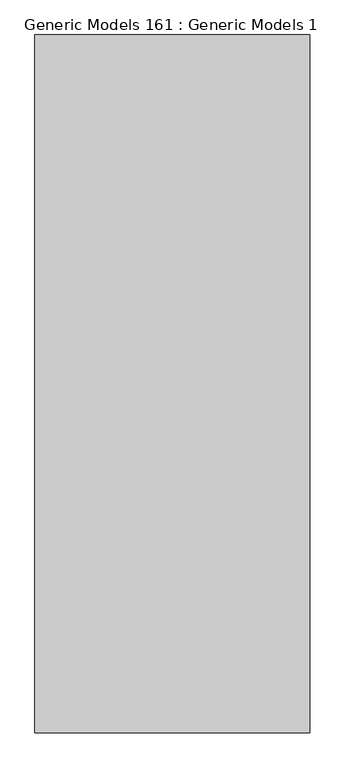
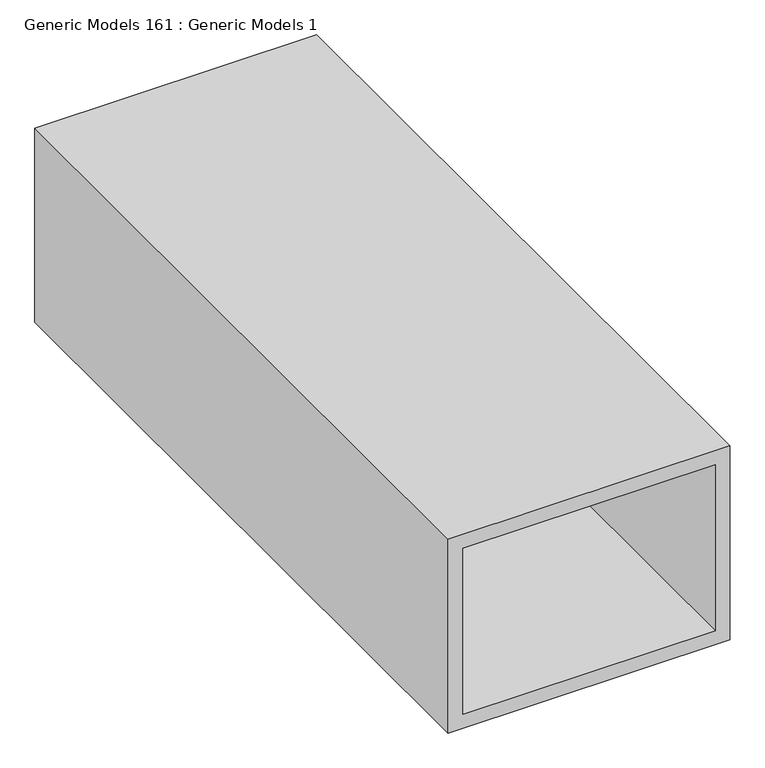
"""IFC4 building model written with IfcOpenShell, lengths in millimetres: proxy geometry, Generic Models 161 : Generic Models 1."""

import ifcopenshell
import ifcopenshell.guid

model = None  # the IFC model being written
_history = None  # IfcOwnerHistory: only IFC2X3 demands one
_inside = {}  # id of a spatial element -> (the spatial element, [elements in it])
_under = {}  # id of a project, library or spatial element -> (it, [spatial elements below it])
_declared = {}  # id of a project -> (the project, [libraries it declares])
_typed = {}  # id of a type object -> (the type object, [elements of that type])
_made_of = {}  # id of a material, layer set ... -> (it, [elements and type objects made of it])


def new_model(schema):
    """Start an empty IFC model of exactly this schema.

    Asked for "IFC4X3", IfcOpenShell would pick the latest addendum, in which some entities
    have other attributes; the version numbers below select the first issue.
    IFC2X3 requires an IfcOwnerHistory on every rooted entity: one is made here for all.
    """
    global model, _history
    if schema == "IFC4X3":
        model = ifcopenshell.file(schema_version=(4, 3, 0, 0))
    else:
        model = ifcopenshell.file(schema=schema)
    _inside.clear()
    _under.clear()
    _declared.clear()
    _typed.clear()
    _made_of.clear()
    _history = None
    if model.schema == "IFC2X3":
        org = make("IfcOrganization", Name="unknown")
        user = make(
            "IfcPersonAndOrganization",
            ThePerson=make("IfcPerson", FamilyName="unknown"),
            TheOrganization=org,
        )
        app = make(
            "IfcApplication",
            ApplicationDeveloper=org,
            Version="unknown",
            ApplicationFullName="unknown",
            ApplicationIdentifier="unknown",
        )
        _history = make(
            "IfcOwnerHistory",
            OwningUser=user,
            OwningApplication=app,
            ChangeAction="ADDED",
            CreationDate=0,
        )
    return model


def make(cls, **values):
    """One entity of the class cls with the attributes given. An attribute that is None is left unset."""
    return model.create_entity(
        cls, **{name: value for name, value in values.items() if value is not None}
    )


def rooted(cls, **values):
    """An entity with a GlobalId (a new one), such as an element, a storey or a relation."""
    return make(cls, GlobalId=ifcopenshell.guid.new(), OwnerHistory=_history, **values)


def si_unit(unit_type, name, prefix=None):
    """IfcSIUnit, for example si_unit("LENGTHUNIT", "METRE", prefix="MILLI")."""
    return make("IfcSIUnit", UnitType=unit_type, Prefix=prefix, Name=name)


def assignment(units):
    """IfcUnitAssignment: the units of a project."""
    return None if units is None else make("IfcUnitAssignment", Units=units)


def point(xyz):
    """IfcCartesianPoint."""
    return None if xyz is None else make("IfcCartesianPoint", Coordinates=xyz)


def direction(xyz):
    """IfcDirection."""
    return None if xyz is None else make("IfcDirection", DirectionRatios=xyz)


def frame(location, z_axis=None, x_axis=None):
    """IfcAxis2Placement3D, a coordinate frame: its origin and axes. An axis left out is left unset."""
    return make(
        "IfcAxis2Placement3D",
        Location=point(location),
        Axis=direction(z_axis),
        RefDirection=direction(x_axis),
    )


def origin():
    """The frame at (0, 0, 0) with its axes left unset."""
    return frame((0.0, 0.0, 0.0))


def place(relative_to, where):
    """IfcLocalPlacement: puts the frame where relative to a parent placement (None: the world)."""
    return make(
        "IfcLocalPlacement", PlacementRelTo=relative_to, RelativePlacement=where
    )


def context(
    kind, dimensions, precision=None, world=None, true_north=None, identifier=None
):
    """IfcGeometricRepresentationContext, for example the 3D "Model" context."""
    return make(
        "IfcGeometricRepresentationContext",
        ContextIdentifier=identifier,
        ContextType=kind,
        CoordinateSpaceDimension=dimensions,
        Precision=precision,
        WorldCoordinateSystem=world,
        TrueNorth=true_north,
    )


def project(units=None, contexts=None):
    """IfcProject with its units and contexts."""
    return rooted(
        "IfcProject",
        Name="project",
        RepresentationContexts=contexts,
        UnitsInContext=assignment(units),
    )


def spatial(cls, under=None, at=None, **own):
    """A site, building, storey or space (cls), placed at a placement, below another one or the project."""
    s = rooted(cls, ObjectPlacement=at, **own)
    if under is not None:
        _under.setdefault(under.id(), (under, []))[1].append(s)
    return s


def polyline(points):
    """IfcPolyline through the points."""
    return make("IfcPolyline", Points=[point(p) for p in points])


def outline(outer, holes=None, kind="AREA"):
    """IfcArbitraryClosedProfileDef: a profile drawn as a closed curve; with holes, ...WithVoids."""
    if holes is None:
        return make("IfcArbitraryClosedProfileDef", ProfileType=kind, OuterCurve=outer)
    return make(
        "IfcArbitraryProfileDefWithVoids",
        ProfileType=kind,
        OuterCurve=outer,
        InnerCurves=holes,
    )


def extrude(swept, where, along, depth):
    """IfcExtrudedAreaSolid: the profile swept, set in the frame where, extruded along a direction by depth."""
    return make(
        "IfcExtrudedAreaSolid",
        SweptArea=swept,
        Position=where,
        ExtrudedDirection=direction(along),
        Depth=depth,
    )


def shape(context_of_items, identifier, shape_type, items):
    """IfcShapeRepresentation: the items that make up one representation, for example the "Body"."""
    return make(
        "IfcShapeRepresentation",
        ContextOfItems=context_of_items,
        RepresentationIdentifier=identifier,
        RepresentationType=shape_type,
        Items=items,
    )


def source(mapping_origin, context_of_items, identifier, shape_type, items):
    """IfcRepresentationMap: a shape defined once, which mapped items show again and again."""
    return make(
        "IfcRepresentationMap",
        MappingOrigin=mapping_origin,
        MappedRepresentation=shape(context_of_items, identifier, shape_type, items),
    )


def transform(
    local_origin,
    x_axis=None,
    y_axis=None,
    z_axis=None,
    scale=None,
    scale2=None,
    scale3=None,
    uniform=True,
):
    """IfcCartesianTransformationOperator3D, or its non-uniform kind. x_axis, y_axis, z_axis: its Axis1, 2, 3."""
    if uniform:
        return make(
            "IfcCartesianTransformationOperator3D",
            Axis1=direction(x_axis),
            Axis2=direction(y_axis),
            LocalOrigin=point(local_origin),
            Scale=scale,
            Axis3=direction(z_axis),
        )
    return make(
        "IfcCartesianTransformationOperator3DnonUniform",
        Axis1=direction(x_axis),
        Axis2=direction(y_axis),
        LocalOrigin=point(local_origin),
        Scale=scale,
        Axis3=direction(z_axis),
        Scale2=scale2,
        Scale3=scale3,
    )


def mapped(mapping_source, mapping_target):
    """IfcMappedItem: shows the shape of a source again, moved by a transform."""
    return make(
        "IfcMappedItem", MappingSource=mapping_source, MappingTarget=mapping_target
    )


def made_of(thing, what):
    """Note that an element or type object is made of a material, layer set ...; save() writes the relation."""
    if what is not None:
        _made_of.setdefault(what.id(), (what, []))[1].append(thing)
    return thing


def element(
    cls,
    number,
    at=None,
    inside=None,
    cuts=None,
    type_object=None,
    material=None,
    context=None,
    identifier="Body",
    shape_type=None,
    held_by="IfcProductDefinitionShape",
    body=None,
    shapes=None,
    **own,
):
    """One element of the class cls, such as IfcWall. Its Tag is "e" and its number.

    at: its placement. inside: the storey or other place that contains it. cuts: it is an
    opening in that element (IfcRelVoidsElement). A single representation is given by context,
    identifier, shape_type and body (its items); several are given by shapes. held_by: the class
    of the entity that holds the representations. save() writes the other relations.
    """
    e = rooted(cls, Tag="e%d" % number, ObjectPlacement=at, **own)
    if body is not None:
        shapes = [shape(context, identifier, shape_type, body)]
    if shapes is not None:
        e.Representation = make(held_by, Representations=shapes)
    if inside is not None:
        _inside.setdefault(inside.id(), (inside, []))[1].append(e)
    if cuts is not None:
        rooted(
            "IfcRelVoidsElement", RelatingBuildingElement=cuts, RelatedOpeningElement=e
        )
    if type_object is not None:
        _typed.setdefault(type_object.id(), (type_object, []))[1].append(e)
    return made_of(e, material)


def aggregate(whole, parts):
    """IfcRelAggregates: a whole, such as a stair, and the parts it consists of."""
    return rooted("IfcRelAggregates", RelatingObject=whole, RelatedObjects=parts)


def save(model, path):
    """Write the relations noted so far, then the file.

    IfcRelAggregates (storeys below a building ...), IfcRelContainedInSpatialStructure (elements
    in a storey), IfcRelDefinesByType, IfcRelAssociatesMaterial and IfcRelDeclares: one each for
    every whole, place, type object, material and project.
    """
    for whole, parts in _under.values():
        aggregate(whole, parts)
    for where, things in _inside.values():
        rooted(
            "IfcRelContainedInSpatialStructure",
            RelatedElements=things,
            RelatingStructure=where,
        )
    for kind, things in _typed.values():
        rooted("IfcRelDefinesByType", RelatedObjects=things, RelatingType=kind)
    for what, things in _made_of.values():
        rooted("IfcRelAssociatesMaterial", RelatedObjects=things, RelatingMaterial=what)
    for by, libraries in _declared.values():
        rooted("IfcRelDeclares", RelatingContext=by, RelatedDefinitions=libraries)
    model.write(path)


def generic_models_161_generic_models_1_b0009ec1(model_context):
    return source(origin(), model_context, "Body", "SweptSolid", [
        extrude(outline(polyline([(2381.25, 51148.3797769), (2381.25, 50668.1069345), (2032.0, 50668.1069345), (2032.0, 51148.3797769), (2381.25, 51148.3797769)]), holes=[polyline([(2355.85, 51122.9797769), (2057.4, 51122.9797769), (2057.4, 50693.5069345), (2355.85, 50693.5069345), (2355.85, 51122.9797769)])]), frame((0.0, 0.0, 0.0), z_axis=(0.0, 1.0, 0.0), x_axis=(0.0, 0.0, 1.0)), (0.0, 0.0, 1.0), 1219.2),
    ])


if __name__ == "__main__":
    model = new_model("IFC4")
    model_context = context("Model", 3, world=origin())
    ifc_project = project(units=[si_unit("LENGTHUNIT", "METRE", prefix="MILLI")], contexts=[model_context])
    site = spatial("IfcSite", under=ifc_project)
    building = spatial("IfcBuilding", under=site)
    placement = place(None, origin())
    generic_models_161_generic_models_1_shape = generic_models_161_generic_models_1_b0009ec1(model_context)
    element("IfcBuildingElementProxy", 1, Name="Generic Models 161 : Generic Models 1", ObjectType="Generic Models 161 : Generic Models 1", at=placement, inside=building, context=model_context, shape_type="MappedRepresentation", body=[
        mapped(generic_models_161_generic_models_1_shape, transform((0.0, 0.0, 0.0), x_axis=(1.0, 0.0, 0.0), y_axis=(0.0, 1.0, 0.0), z_axis=(0.0, 0.0, 1.0))),
    ])
    save(model, "model.ifc")

# Revit data of these elements
# Element 1 (IfcBuildingElementProxy, "Generic Models 161 : Generic Models 1")
#   Materials on its faces: "IF THERE'S AN OPEN AIR WAY PATH, THROUGH THE DUCTS, FROM ONE ROOM TO THE OTHER, EITHER 1)LINE THE INTERIOR OF THE DUCT W/ SOUNDABSORPTIVE MATERIAL AND/OR 2) USE A 'DUCT BAFFLE BOX' TO MUFFLE THE MIGRATING SOUND"
# Materials
#   "IF THERE'S AN OPEN AIR WAY PATH, THROUGH THE DUCTS, FROM ONE ROOM TO THE OTHER, EITHER 1)LINE THE INTERIOR OF THE DUCT W/ SOUNDABSORPTIVE MATERIAL AND/OR 2) USE A 'DUCT BAFFLE BOX' TO MUFFLE THE MIGRATING SOUND": class "Generic", colour RGB 127 127 127, transparency 0, Description = "Rigid foam insulation board", Cost = 0
